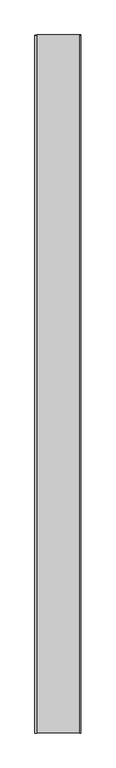
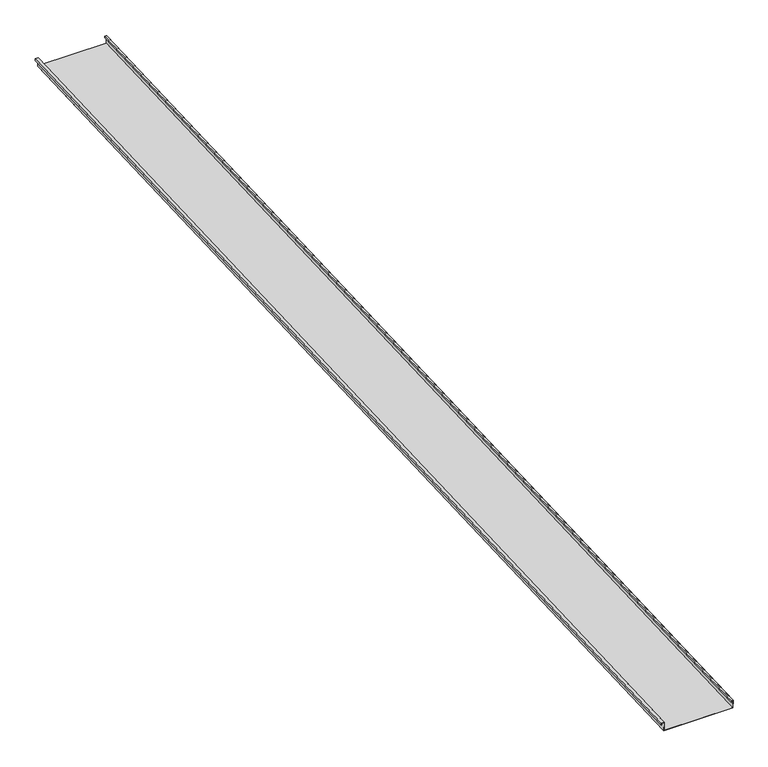
"""IFC4 building model written with IfcOpenShell, lengths in millimetres: proxy geometry, Generic Models 2:Generic Models 2:310765:Generic Models 2:310765 : Generic Models 2:Generic Models 2:310765:132 : Generic Models 2:Generic Models 2:310765:Generic Models 2:310765 : Generic Models 2:Generic Models 2:310765:300385."""

from ifc_helpers import new_model, si_unit, frame, origin, place, context, project, spatial, polyline, outline, extrude, source, transform, mapped, element, save


def generic_models_3ef2793e(model_context):
    return source(origin(), model_context, "Body", "SweptSolid", [
        extrude(outline(polyline([(1.5875, 0.0), (1.5875, 50.8), (407.9875, 50.8), (407.9875, 1.5875), (396.875, 1.5875), (396.875, 11.1125), (398.4625, 11.1125), (398.4625, 3.175), (406.4, 3.175), (406.4, 49.2125), (3.175, 49.2125), (3.175, -1.5874999), (-14.2875, -1.5874999), (-14.2875, 9.525), (-12.7, 9.525), (-12.7, 0.0), (1.5875, 0.0)])), frame((659715.9096405, -581354.4345603, 3902.6697972), z_axis=(0.0, 0.9991330730923568, 0.041630544712067834), x_axis=(1.0, 0.0, 0.0)), (0.0, 0.0, 1.0), 6400.8),
    ])


if __name__ == "__main__":
    model = new_model("IFC4")
    model_context = context("Model", 3, world=origin())
    ifc_project = project(units=[si_unit("LENGTHUNIT", "METRE", prefix="MILLI")], contexts=[model_context])
    site = spatial("IfcSite", under=ifc_project)
    building = spatial("IfcBuilding", under=site)
    placement = place(None, origin())
    generic_models_shape = generic_models_3ef2793e(model_context)
    element("IfcBuildingElementProxy", 1, Name="Generic Models 2:Generic Models 2:310765:Generic Models 2:310765 : Generic Models 2:Generic Models 2:310765:132 : Generic Models 2:Generic Models 2:310765:Generic Models 2:310765 : Generic Models 2:Generic Models 2:310765:300385", ObjectType="Generic Models 2:Generic Models 2:310765:Generic Models 2:310765 : Generic Models 2:Generic Models 2:310765:132 : Generic Models 2:Generic Models 2:310765:Generic Models 2:310765 : Generic Models 2:Generic Models 2:310765:300385", at=placement, inside=building, context=model_context, shape_type="MappedRepresentation", body=[
        mapped(generic_models_shape, transform((0.0, 0.0, 0.0), x_axis=(1.0, 0.0, 0.0), y_axis=(0.0, 1.0, 0.0), z_axis=(0.0, 0.0, 1.0))),
    ])
    save(model, "model.ifc")

# Revit data of these elements
# Type "Generic Models 2:Generic Models 2:310765:Generic Models 2:310765 : Generic Models 2:Generic Models 2:310765:132 : Generic Models 2:Generic Models 2:310765:Generic Models 2:310765 : Generic Models 2:Generic Models 2:310765:300385"
#   NameOverride = "Generic Models 2:Generic Models 2:310765:Generic Models 2:310765 : Generic Models 2:Generic Models 2:310765:300385"
#   ObjectTypeOverride = "Generic Models 2:310765 : Generic Models 2:Generic Models 2:310765"
#   Reference = "Generic Models 2"
#   Tag = "300385"
# Element 1 (IfcBuildingElementProxy, "Generic Models 2:Generic Models 2:310765:Generic Models 2:310765 : Generic Models 2:Generic Models 2:310765:132 : Generic Models 2:Generic Models 2:310765:Generic Models 2:310765 : Generic Models 2:Generic Models 2:310765:300385")
#   Materials on its faces: "THERMAL BROKEN ALUMINUM STOREFRONT FOR POLYCARBONATE"
# Materials
#   "THERMAL BROKEN ALUMINUM STOREFRONT FOR POLYCARBONATE": class "Unassigned", colour RGB 244 244 244, transparency 0, Keynote = "M07611300.01", Cost = 0
